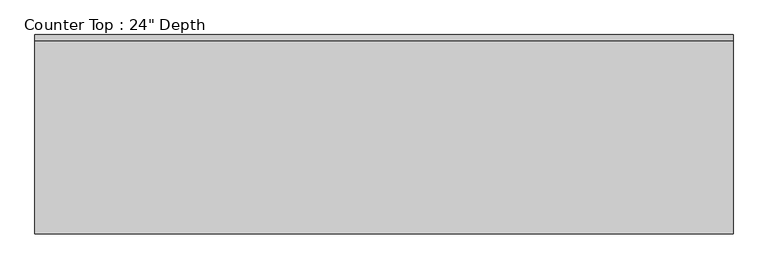
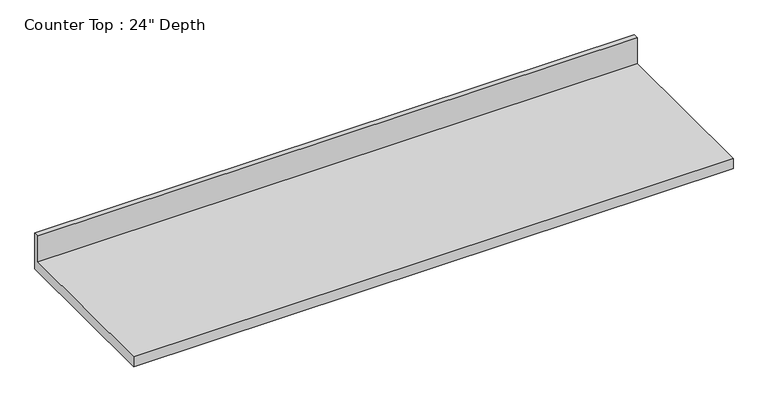
"""IFC4 building model written with IfcOpenShell, lengths in millimetres: furniture geometry."""

from ifc_helpers import new_model, si_unit, frame, origin, place, context, project, spatial, polyline, outline, extrude, source, transform, mapped, element, save


def furniture_6bf0da8d(model_context):
    return source(origin(), model_context, "Body", "SweptSolid", [
        extrude(outline(polyline([(0.0, 1016.0), (0.0, 876.3), (-635.0, 876.3), (-635.0, 914.4), (-19.05, 914.4), (-19.05, 1016.0), (0.0, 1016.0)])), frame((-1200.4622951, 0.0, 0.0), z_axis=(1.0, 0.0, 0.0), x_axis=(0.0, 1.0, 0.0)), (0.0, 0.0, 1.0), 2224.0875),
    ])


if __name__ == "__main__":
    model = new_model("IFC4")
    model_context = context("Model", 3, world=origin())
    ifc_project = project(units=[si_unit("LENGTHUNIT", "METRE", prefix="MILLI")], contexts=[model_context])
    site = spatial("IfcSite", under=ifc_project)
    building = spatial("IfcBuilding", under=site)
    placement = place(None, origin())
    furniture_shape = furniture_6bf0da8d(model_context)
    element("IfcFurniture", 1, ObjectType="Counter Top : 24\" Depth", at=placement, inside=building, context=model_context, shape_type="MappedRepresentation", body=[
        mapped(furniture_shape, transform((0.0, 0.0, 0.0), x_axis=(1.0, 0.0, 0.0), y_axis=(0.0, 1.0, 0.0), z_axis=(0.0, 0.0, 1.0))),
    ])
    save(model, "model.ifc")

# Revit data of these elements
# Type "Counter Top : 24\" Depth"
#   Assembly Code = "C1030400"
#   Counter Thickness = 0' - 1 1/2"
#   Depth = 2' - 1"
#   Height = 3' - 0"
#   Length [instance default] = 8' - 0"
#   Counter Top Material = none
#   Default Elevation = 0
# Element 1 (IfcFurniture, "Counter Top : 24\" Depth")
#   Length = 7' - 3 9/16"
#   Materials on its faces: "Counter Top"
# Materials
#   "Counter Top": class "Wood", colour RGB 226 177 128, transparency 0
